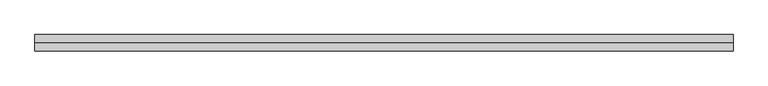
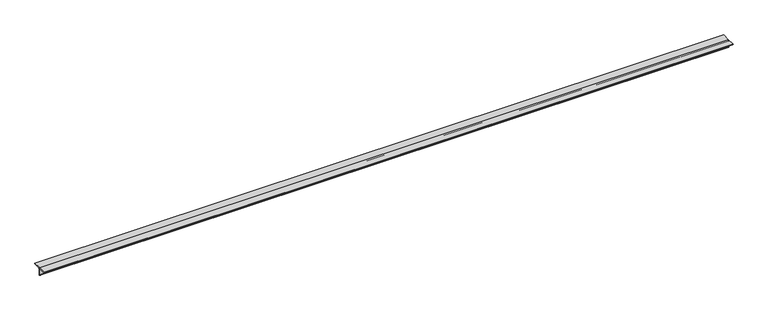
"""IFC4 building model written with IfcOpenShell, lengths in millimetres: member geometry, 0123_Steel Framing_2Ls-KSD3502 : H_SB_AR_S03_2Ls-130x130x12_HBR1."""

from ifc_helpers import new_model, si_unit, point, frame, frame_2d, origin, place, context, project, spatial, polyline, circle_curve, trimmed, segment, composite_curve, outline, extrude, source, transform, mapped, element, save


def member_4dd44919(model_context):
    return source(origin(), model_context, "Body", "SweptSolid", [
        extrude(outline(composite_curve([segment(polyline([(0.0, 36.4), (0.0, -93.6)]), True, "CONTINUOUS"), segment(trimmed(circle_curve(frame_2d((0.0, -81.6)), 12.0), [point((0.0, -93.6))], [point((-12.0, -81.6))], False, "CARTESIAN"), True, "CONTINUOUS"), segment(polyline([(-12.0, -81.6), (-12.0, 12.4)]), True, "CONTINUOUS"), segment(trimmed(circle_curve(frame_2d((-24.0, 12.4)), 12.0), [point((-12.0, 12.4))], [point((-24.0, 24.4))], True, "CARTESIAN"), True, "CONTINUOUS"), segment(polyline([(-24.0, 24.4), (-118.0, 24.4)]), True, "CONTINUOUS"), segment(trimmed(circle_curve(frame_2d((-118.0, 36.4)), 12.0), [point((-118.0, 24.4))], [point((-130.0, 36.4))], False, "CARTESIAN"), True, "CONTINUOUS"), segment(polyline([(-130.0, 36.4), (0.0, 36.4)]), True, "CONTINUOUS")], self_intersect=False)), frame((-5571.7417611, 0.0, 0.0), z_axis=(1.0, 0.0, 0.0), x_axis=(0.0, 1.0, 0.0)), (0.0, 0.0, 1.0), 11162.5198652),
        extrude(outline(composite_curve([segment(polyline([(0.0, 36.4), (130.0, 36.4)]), True, "CONTINUOUS"), segment(trimmed(circle_curve(frame_2d((118.0, 36.4)), 12.0), [point((130.0, 36.4))], [point((118.0, 24.4))], False, "CARTESIAN"), True, "CONTINUOUS"), segment(polyline([(118.0, 24.4), (24.0, 24.4)]), True, "CONTINUOUS"), segment(trimmed(circle_curve(frame_2d((24.0, 12.4)), 12.0), [point((24.0, 24.4))], [point((12.0, 12.4))], True, "CARTESIAN"), True, "CONTINUOUS"), segment(polyline([(12.0, 12.4), (12.0, -81.6)]), True, "CONTINUOUS"), segment(trimmed(circle_curve(frame_2d((0.0, -81.6)), 12.0), [point((12.0, -81.6))], [point((0.0, -93.6))], False, "CARTESIAN"), True, "CONTINUOUS"), segment(polyline([(0.0, -93.6), (0.0, 36.4)]), True, "CONTINUOUS")], self_intersect=False)), frame((-5571.7417611, 0.0, 0.0), z_axis=(1.0, 0.0, 0.0), x_axis=(0.0, 1.0, 0.0)), (0.0, 0.0, 1.0), 11162.5198652),
    ])


if __name__ == "__main__":
    model = new_model("IFC4")
    model_context = context("Model", 3, world=origin())
    ifc_project = project(units=[si_unit("LENGTHUNIT", "METRE", prefix="MILLI")], contexts=[model_context])
    site = spatial("IfcSite", under=ifc_project)
    building = spatial("IfcBuilding", under=site)
    placement = place(None, origin())
    member_shape = member_4dd44919(model_context)
    element("IfcMember", 1, ObjectType="0123_Steel Framing_2Ls-KSD3502 : H_SB_AR_S03_2Ls-130x130x12_HBR1", at=placement, inside=building, context=model_context, shape_type="MappedRepresentation", body=[
        mapped(member_shape, transform((0.0, 0.0, 0.0), x_axis=(1.0, 0.0, 0.0), y_axis=(0.0, 1.0, 0.0), z_axis=(0.0, 0.0, 1.0))),
    ])
    save(model, "model.ifc")

# Revit data of these elements
# Type "0123_Steel Framing_2Ls-KSD3502 : H_SB_AR_S03_2Ls-130x130x12_HBR1"
#   Type Mark = "HBR1"
#   Assembly Code = "B10"
#   Legs = "SLBB"
#   W = 8.97
#   Perimeter = 1.04 m²/m
#   Nominal Weight = 46.80 kgf/m
#   Length [instance default] = 1000 mm
#   Space = 0 mm
#   b = 130 mm
#   d = 130 mm
#   t = 12 mm
#   y = 36.4 mm
#   A = 0.005952 m²
#   Structural Material [instance default] = Steel ASTM A36
# Element 1 (IfcMember, "0123_Steel Framing_2Ls-KSD3502 : H_SB_AR_S03_2Ls-130x130x12_HBR1")
#   Materials on its faces: "Steel ASTM A36"
# Materials
#   "Steel ASTM A36": class "Metal", colour RGB 199 199 199, transparency 0, Description = "Structural steel, ASTM A36 Grade B, mill finish", Cost = 0
